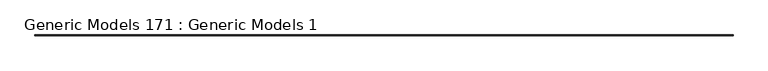
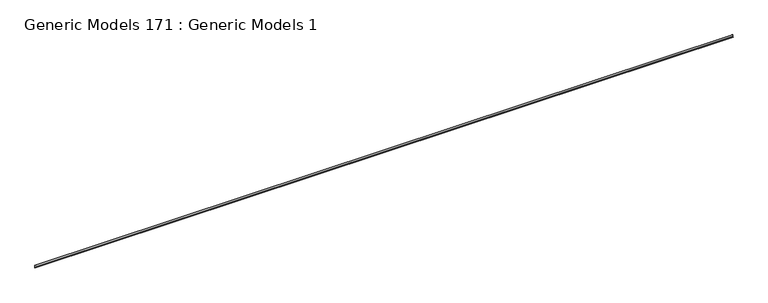
"""IFC4 building model written with IfcOpenShell, lengths in millimetres: proxy geometry, Generic Models 171 : Generic Models 1."""

from ifc_helpers import new_model, si_unit, frame, origin, place, context, project, spatial, polyline, outline, extrude, source, transform, mapped, element, save


def generic_models_171_generic_models_1_b43b51aa(model_context):
    return source(origin(), model_context, "Body", "SweptSolid", [
        extrude(outline(polyline([(-5493.3230338, 126975.1083131), (-5472.3680338, 126981.8438488), (-5472.3680338, 127025.9083131), (-5471.0980338, 127025.9083131), (-5471.0980338, 126980.9180695), (-5489.1728315, 126975.1083131), (-5472.0612289, 126969.6081551), (-5471.0980338, 126964.4934048), (-5472.3460963, 126964.2583732), (-5473.1694173, 126968.630365), (-5493.3230338, 126975.1083131)])), frame((-16853.0736296, 0.0, 0.0), z_axis=(1.0, 0.0, 0.0), x_axis=(0.0, 1.0, 0.0)), (0.0, 0.0, 1.0), 19050.0),
    ])


if __name__ == "__main__":
    model = new_model("IFC4")
    model_context = context("Model", 3, world=origin())
    ifc_project = project(units=[si_unit("LENGTHUNIT", "METRE", prefix="MILLI")], contexts=[model_context])
    site = spatial("IfcSite", under=ifc_project)
    building = spatial("IfcBuilding", under=site)
    placement = place(None, origin())
    generic_models_171_generic_models_1_shape = generic_models_171_generic_models_1_b43b51aa(model_context)
    element("IfcBuildingElementProxy", 1, Name="Generic Models 171 : Generic Models 1", ObjectType="Generic Models 171 : Generic Models 1", at=placement, inside=building, context=model_context, shape_type="MappedRepresentation", body=[
        mapped(generic_models_171_generic_models_1_shape, transform((0.0, 0.0, 0.0), x_axis=(1.0, 0.0, 0.0), y_axis=(0.0, 1.0, 0.0), z_axis=(0.0, 0.0, 1.0))),
    ])
    save(model, "model.ifc")

# Revit data of these elements
# Element 1 (IfcBuildingElementProxy, "Generic Models 171 : Generic Models 1")
#   Materials on its faces: "_16 GA. COPPER WEEP SCREED W/ MIN. 3 1/2\" ATTACHEMENT FLANGE - LAP UNDERLAYMENT OVER WEED SCREED"
# Materials
#   "_16 GA. COPPER WEEP SCREED W/ MIN. 3 1/2\" ATTACHEMENT FLANGE - LAP UNDERLAYMENT OVER WEED SCREED": class "Generic", colour RGB 253 192 103, transparency 0, Cost = 0
